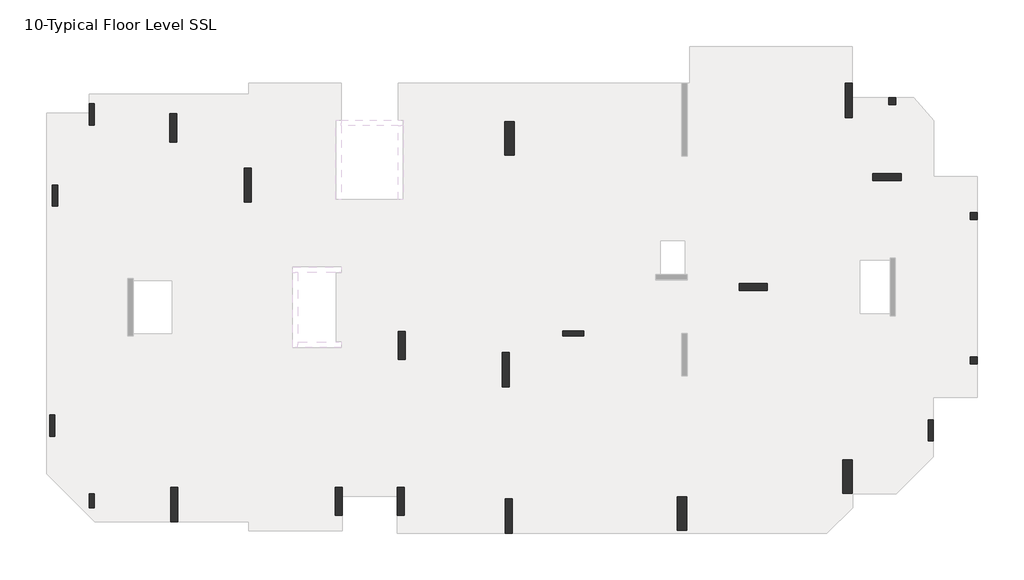
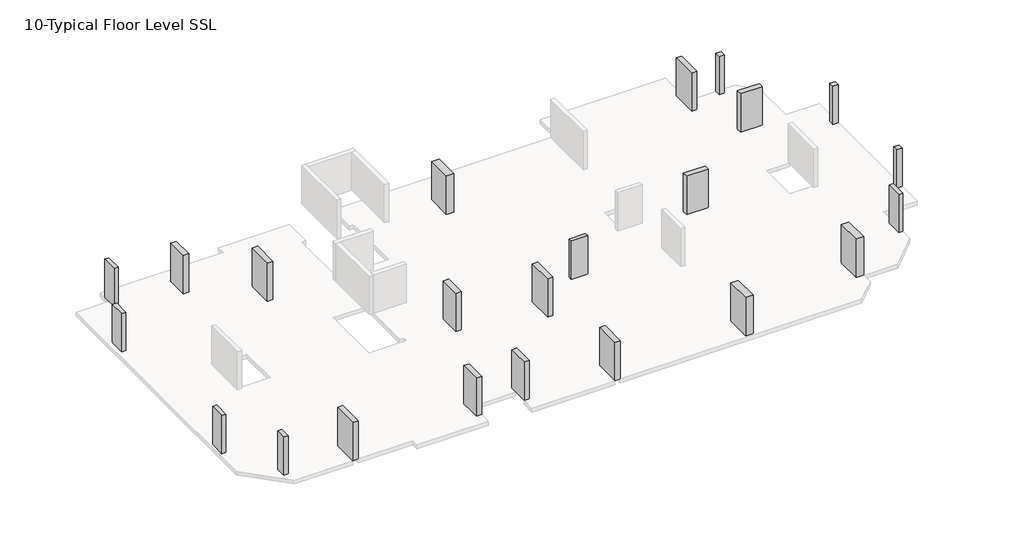
# One storey, part 2 of 2: 23 columns.
"""IFC4 building model written with IfcOpenShell, lengths in millimetres."""

import ifcopenshell
import ifcopenshell.guid

model = None  # the IFC model being written
_history = None  # IfcOwnerHistory: only IFC2X3 demands one
_inside = {}  # id of a spatial element -> (the spatial element, [elements in it])
_under = {}  # id of a project, library or spatial element -> (it, [spatial elements below it])
_declared = {}  # id of a project -> (the project, [libraries it declares])
_typed = {}  # id of a type object -> (the type object, [elements of that type])
_made_of = {}  # id of a material, layer set ... -> (it, [elements and type objects made of it])


def new_model(schema):
    """Start an empty IFC model of exactly this schema.

    Asked for "IFC4X3", IfcOpenShell would pick the latest addendum, in which some entities
    have other attributes; the version numbers below select the first issue.
    IFC2X3 requires an IfcOwnerHistory on every rooted entity: one is made here for all.
    """
    global model, _history
    if schema == "IFC4X3":
        model = ifcopenshell.file(schema_version=(4, 3, 0, 0))
    else:
        model = ifcopenshell.file(schema=schema)
    _inside.clear()
    _under.clear()
    _declared.clear()
    _typed.clear()
    _made_of.clear()
    _history = None
    if model.schema == "IFC2X3":
        org = make("IfcOrganization", Name="unknown")
        user = make(
            "IfcPersonAndOrganization",
            ThePerson=make("IfcPerson", FamilyName="unknown"),
            TheOrganization=org,
        )
        app = make(
            "IfcApplication",
            ApplicationDeveloper=org,
            Version="unknown",
            ApplicationFullName="unknown",
            ApplicationIdentifier="unknown",
        )
        _history = make(
            "IfcOwnerHistory",
            OwningUser=user,
            OwningApplication=app,
            ChangeAction="ADDED",
            CreationDate=0,
        )
    return model


def make(cls, **values):
    """One entity of the class cls with the attributes given. An attribute that is None is left unset."""
    return model.create_entity(
        cls, **{name: value for name, value in values.items() if value is not None}
    )


def rooted(cls, **values):
    """An entity with a GlobalId (a new one), such as an element, a storey or a relation."""
    return make(cls, GlobalId=ifcopenshell.guid.new(), OwnerHistory=_history, **values)


def si_unit(unit_type, name, prefix=None):
    """IfcSIUnit, for example si_unit("LENGTHUNIT", "METRE", prefix="MILLI")."""
    return make("IfcSIUnit", UnitType=unit_type, Prefix=prefix, Name=name)


def assignment(units):
    """IfcUnitAssignment: the units of a project."""
    return None if units is None else make("IfcUnitAssignment", Units=units)


def point(xyz):
    """IfcCartesianPoint."""
    return None if xyz is None else make("IfcCartesianPoint", Coordinates=xyz)


def direction(xyz):
    """IfcDirection."""
    return None if xyz is None else make("IfcDirection", DirectionRatios=xyz)


def frame(location, z_axis=None, x_axis=None):
    """IfcAxis2Placement3D, a coordinate frame: its origin and axes. An axis left out is left unset."""
    return make(
        "IfcAxis2Placement3D",
        Location=point(location),
        Axis=direction(z_axis),
        RefDirection=direction(x_axis),
    )


def origin():
    """The frame at (0, 0, 0) with its axes left unset."""
    return frame((0.0, 0.0, 0.0))


def place(relative_to, where):
    """IfcLocalPlacement: puts the frame where relative to a parent placement (None: the world)."""
    return make(
        "IfcLocalPlacement", PlacementRelTo=relative_to, RelativePlacement=where
    )


def context(
    kind, dimensions, precision=None, world=None, true_north=None, identifier=None
):
    """IfcGeometricRepresentationContext, for example the 3D "Model" context."""
    return make(
        "IfcGeometricRepresentationContext",
        ContextIdentifier=identifier,
        ContextType=kind,
        CoordinateSpaceDimension=dimensions,
        Precision=precision,
        WorldCoordinateSystem=world,
        TrueNorth=true_north,
    )


def project(units=None, contexts=None):
    """IfcProject with its units and contexts."""
    return rooted(
        "IfcProject",
        Name="project",
        RepresentationContexts=contexts,
        UnitsInContext=assignment(units),
    )


def spatial(cls, under=None, at=None, **own):
    """A site, building, storey or space (cls), placed at a placement, below another one or the project."""
    s = rooted(cls, ObjectPlacement=at, **own)
    if under is not None:
        _under.setdefault(under.id(), (under, []))[1].append(s)
    return s


def faces_of(points, faces, orient=None, outer=None):
    """IfcFace entities. A face is a list of loops; a loop is a list of indices into points, from 0.

    orient and outer hold one flag for each loop. By default every Orientation is true, the
    first loop of a face is its IfcFaceOuterBound and the others are IfcFaceBound.
    """
    made = []
    for i, loops in enumerate(faces):
        bounds = []
        for j, loop in enumerate(loops):
            is_outer = j == 0 if outer is None else outer[i][j]
            bounds.append(
                make(
                    "IfcFaceOuterBound" if is_outer else "IfcFaceBound",
                    Bound=make("IfcPolyLoop", Polygon=[points[k] for k in loop]),
                    Orientation=True if orient is None else orient[i][j],
                )
            )
        made.append(make("IfcFace", Bounds=bounds))
    return made


def faceted_brep(points, faces, orient=None, outer=None, voids=None):
    """IfcFacetedBrep: a solid bounded by flat faces; with voids (closed shells), ...WithVoids."""
    shared = [point(p) for p in points]
    hull = make("IfcClosedShell", CfsFaces=faces_of(shared, faces, orient, outer))
    if voids is None:
        return make("IfcFacetedBrep", Outer=hull)
    return make(
        "IfcFacetedBrepWithVoids",
        Outer=hull,
        Voids=[
            make(cls, CfsFaces=faces_of(shared, fs, o, b)) for cls, fs, o, b in voids
        ],
    )


def shape(context_of_items, identifier, shape_type, items):
    """IfcShapeRepresentation: the items that make up one representation, for example the "Body"."""
    return make(
        "IfcShapeRepresentation",
        ContextOfItems=context_of_items,
        RepresentationIdentifier=identifier,
        RepresentationType=shape_type,
        Items=items,
    )


def made_of(thing, what):
    """Note that an element or type object is made of a material, layer set ...; save() writes the relation."""
    if what is not None:
        _made_of.setdefault(what.id(), (what, []))[1].append(thing)
    return thing


def element(
    cls,
    number,
    at=None,
    inside=None,
    cuts=None,
    type_object=None,
    material=None,
    context=None,
    identifier="Body",
    shape_type=None,
    held_by="IfcProductDefinitionShape",
    body=None,
    shapes=None,
    **own,
):
    """One element of the class cls, such as IfcWall. Its Tag is "e" and its number.

    at: its placement. inside: the storey or other place that contains it. cuts: it is an
    opening in that element (IfcRelVoidsElement). A single representation is given by context,
    identifier, shape_type and body (its items); several are given by shapes. held_by: the class
    of the entity that holds the representations. save() writes the other relations.
    """
    e = rooted(cls, Tag="e%d" % number, ObjectPlacement=at, **own)
    if body is not None:
        shapes = [shape(context, identifier, shape_type, body)]
    if shapes is not None:
        e.Representation = make(held_by, Representations=shapes)
    if inside is not None:
        _inside.setdefault(inside.id(), (inside, []))[1].append(e)
    if cuts is not None:
        rooted(
            "IfcRelVoidsElement", RelatingBuildingElement=cuts, RelatedOpeningElement=e
        )
    if type_object is not None:
        _typed.setdefault(type_object.id(), (type_object, []))[1].append(e)
    return made_of(e, material)


def aggregate(whole, parts):
    """IfcRelAggregates: a whole, such as a stair, and the parts it consists of."""
    return rooted("IfcRelAggregates", RelatingObject=whole, RelatedObjects=parts)


def save(model, path):
    """Write the relations noted so far, then the file.

    IfcRelAggregates (storeys below a building ...), IfcRelContainedInSpatialStructure (elements
    in a storey), IfcRelDefinesByType, IfcRelAssociatesMaterial and IfcRelDeclares: one each for
    every whole, place, type object, material and project.
    """
    for whole, parts in _under.values():
        aggregate(whole, parts)
    for where, things in _inside.values():
        rooted(
            "IfcRelContainedInSpatialStructure",
            RelatedElements=things,
            RelatingStructure=where,
        )
    for kind, things in _typed.values():
        rooted("IfcRelDefinesByType", RelatedObjects=things, RelatingType=kind)
    for what, things in _made_of.values():
        rooted("IfcRelAssociatesMaterial", RelatedObjects=things, RelatingMaterial=what)
    for by, libraries in _declared.values():
        rooted("IfcRelDeclares", RelatingContext=by, RelatedDefinitions=libraries)
    model.write(path)


model = new_model("IFC4")

# Units and contexts
model_context = context("Model", 3, world=origin())
ifc_project = project(units=[si_unit("LENGTHUNIT", "METRE", prefix="MILLI")], contexts=[model_context])

# Site, building, storey
site = spatial("IfcSite", under=ifc_project)
building = spatial("IfcBuilding", under=site)
storey = spatial("IfcBuildingStorey", under=building, Name="10-Typical Floor Level SSL", Elevation=24000.0)

# Columns
placement = place(None, origin())
element("IfcColumn", 1, ObjectType="M_Concrete-Rectangular-Column : C-1 (400 x 400mm)", at=placement, inside=storey, context=model_context, shape_type="Brep", body=[
    faceted_brep([(52549.9999998, 16712.0, 24000.0), (52549.9999998, 16312.0, 24000.0), (52149.9999998, 16312.0, 24000.0), (52149.9999998, 16712.0, 24000.0), (52549.9999998, 16712.0, 27000.0), (52549.9999998, 16312.0, 27000.0), (52549.9999998, 16312.0, 26700.0), (52549.9999998, 16712.0, 26700.0), (52149.9999998, 16312.0, 27000.0), (52149.9999998, 16312.0, 26700.0), (52149.9999998, 16712.0, 27000.0), (52149.9999998, 16712.0, 26700.0)], [[[0, 1, 2, 3]], [[4, 5, 6, 1, 0, 7]], [[5, 8, 9, 2, 1, 6]], [[8, 10, 11, 3, 2, 9]], [[10, 4, 7, 0, 3, 11]], [[4, 10, 8, 5]]]),
])
element("IfcColumn", 2, ObjectType="M_Concrete-Rectangular-Column : C-1 (400 x 400mm)", at=placement, inside=storey, context=model_context, shape_type="Brep", body=[
    faceted_brep([(47898.6337868, 23252.0, 24000.0), (47898.6337868, 22852.0, 24000.0), (47498.6337868, 22852.0, 24000.0), (47498.6337868, 23252.0, 24000.0), (47898.6337868, 23252.0, 27000.0), (47898.6337868, 22852.0, 27000.0), (47898.6337868, 22852.0, 26700.0), (47498.6337868, 22852.0, 27000.0), (47498.6337868, 22852.0, 26700.0), (47498.6337868, 23252.0, 27000.0)], [[[0, 1, 2, 3]], [[4, 5, 6, 1, 0]], [[5, 7, 8, 2, 1, 6]], [[7, 9, 3, 2, 8]], [[9, 4, 0, 3]], [[4, 9, 7, 5]]]),
])
element("IfcColumn", 3, ObjectType="M_Concrete-Rectangular-Column : C-1 (400 x 400mm)", at=placement, inside=storey, context=model_context, shape_type="Brep", body=[
    faceted_brep([(52549.9999998, 8504.0039609, 24000.0), (52549.9999998, 8104.0039609, 24000.0), (52149.9999998, 8104.0039609, 24000.0), (52149.9999998, 8504.0039609, 24000.0), (52549.9999998, 8504.0039609, 27000.0), (52549.9999998, 8104.0039609, 27000.0), (52549.9999998, 8104.0039609, 26700.0), (52549.9999998, 8504.0039609, 26700.0), (52149.9999998, 8104.0039609, 27000.0), (52149.9999998, 8104.0039609, 26700.0), (52149.9999998, 8504.0039609, 27000.0), (52149.9999998, 8504.0039609, 26700.0)], [[[0, 1, 2, 3]], [[4, 5, 6, 1, 0, 7]], [[5, 8, 9, 2, 1, 6]], [[8, 10, 11, 3, 2, 9]], [[10, 4, 7, 0, 3, 11]], [[4, 10, 8, 5]]]),
])
element("IfcColumn", 4, ObjectType="M_Concrete-Rectangular-Column : C-2 (300 x 800mm)", at=placement, inside=storey, context=model_context, shape_type="Brep", body=[
    faceted_brep([(2352.0, 728.0, 24000.0), (2352.0, -72.0, 24000.0), (2052.0, -72.0, 24000.0), (2052.0, 728.0, 24000.0), (2352.0, 728.0, 27000.0), (2352.0, -72.0, 27000.0), (2352.0, -72.0, 26700.0), (2352.0, 728.0, 26700.0), (2052.0, -72.0, 27000.0), (2052.0, -72.0, 26700.0), (2052.0, 728.0, 27000.0), (2052.0, 728.0, 26700.0)], [[[0, 1, 2, 3]], [[4, 5, 6, 1, 0, 7]], [[5, 8, 9, 2, 1, 6]], [[8, 10, 11, 3, 2, 9]], [[10, 4, 7, 0, 3, 11]], [[4, 10, 8, 5]]]),
])
element("IfcColumn", 5, ObjectType="M_Concrete-Rectangular-Column : C-3(300 x 1200mm)", at=placement, inside=storey, context=model_context, shape_type="Brep", body=[
    faceted_brep([(2352.0, 22908.0000656, 24000.0), (2352.0, 21708.0000656, 24000.0), (2052.0, 21708.0000656, 24000.0), (2052.0, 22908.0000656, 24000.0), (2352.0, 22908.0000656, 27000.0), (2352.0, 21708.0000656, 27000.0), (2352.0, 21708.0000656, 26700.0), (2352.0, 22908.0000656, 26700.0), (2052.0, 21708.0000656, 27000.0), (2052.0, 21708.0000656, 26700.0), (2052.0, 22380.0004589, 27000.0), (2052.0, 22908.0000656, 27000.0), (2052.0, 22908.0000656, 26700.0)], [[[0, 1, 2, 3]], [[4, 5, 6, 1, 0, 7]], [[5, 8, 9, 2, 1, 6]], [[8, 10, 11, 12, 3, 2, 9]], [[11, 4, 7, 0, 3, 12]], [[4, 11, 10, 8, 5]]]),
])
element("IfcColumn", 6, ObjectType="M_Concrete-Rectangular-Column : C-3(300 x 1200mm)", at=placement, inside=storey, context=model_context, shape_type="Brep", body=[
    faceted_brep([(257.9999999, 18288.0, 24000.0), (257.9999999, 17088.0, 24000.0), (-42.0000001, 17088.0, 24000.0), (-42.0000001, 18288.0, 24000.0), (257.9999999, 18288.0, 27000.0), (257.9999999, 17088.0, 27000.0), (257.9999999, 17088.0, 26700.0), (257.9999999, 18288.0, 26700.0), (-42.0000001, 17088.0, 27000.0), (-42.0000001, 17088.0, 26700.0), (-42.0000001, 18288.0, 27000.0), (-42.0000001, 18288.0, 26700.0)], [[[0, 1, 2, 3]], [[4, 5, 6, 1, 0, 7]], [[5, 8, 9, 2, 1, 6]], [[8, 10, 11, 3, 2, 9]], [[10, 4, 7, 0, 3, 11]], [[4, 10, 8, 5]]]),
])
element("IfcColumn", 7, ObjectType="M_Concrete-Rectangular-Column : C-3(300 x 1200mm)", at=placement, inside=storey, context=model_context, shape_type="Brep", body=[
    faceted_brep([(108.001803, 5201.9999858, 24000.0), (108.001803, 4001.9999858, 24000.0), (-191.998197, 4001.9999858, 24000.0), (-191.998197, 5201.9999858, 24000.0), (108.001803, 5201.9999858, 27000.0), (108.001803, 4001.9999858, 27000.0), (108.001803, 4001.9999858, 26700.0), (108.001803, 5201.9999858, 26700.0), (-191.998197, 4001.9999858, 27000.0), (-191.998197, 4001.9999858, 26700.0), (-191.998197, 5201.9999858, 27000.0), (-191.998197, 5201.9999858, 26700.0)], [[[0, 1, 2, 3]], [[4, 5, 6, 1, 0, 7]], [[5, 8, 9, 2, 1, 6]], [[8, 10, 11, 3, 2, 9]], [[10, 4, 7, 0, 3, 11]], [[4, 10, 8, 5]]]),
])
element("IfcColumn", 8, ObjectType="M_Concrete-Rectangular-Column : C-3(300 x 1200mm)", at=placement, inside=storey, context=model_context, shape_type="Brep", body=[
    faceted_brep([(50046.0009271, 4931.9999929, 24000.0), (50046.0009271, 3731.9999929, 24000.0), (49746.0009271, 3731.9999929, 24000.0), (49746.0009271, 4931.9999929, 24000.0), (50046.0009271, 4931.9999929, 27000.0), (50046.0009271, 3731.9999929, 27000.0), (50046.0009271, 3731.9999929, 26700.0), (50046.0009271, 4931.9999929, 26700.0), (49746.0009271, 3731.9999929, 27000.0), (49746.0009271, 3731.9999929, 26700.0), (49746.0009271, 4931.9999929, 27000.0), (49746.0009271, 4931.9999929, 26700.0)], [[[0, 1, 2, 3]], [[4, 5, 6, 1, 0, 7]], [[5, 8, 9, 2, 1, 6]], [[8, 10, 11, 3, 2, 9]], [[10, 4, 7, 0, 3, 11]], [[4, 10, 8, 5]]]),
])
element("IfcColumn", 9, ObjectType="M_Concrete-Rectangular-Column : C-3(300 x 1200mm)", at=placement, inside=storey, context=model_context, shape_type="Brep", body=[
    faceted_brep([(28975.9999998, 9996.0000019, 24000.0), (30175.9999998, 9996.0000019, 24000.0), (30175.9999998, 9696.0000019, 24000.0), (28975.9999998, 9696.0000019, 24000.0), (28975.9999998, 9996.0000019, 27000.0), (30175.9999998, 9996.0000019, 27000.0), (30175.9999998, 9996.0000019, 26700.0), (28975.9999998, 9996.0000019, 26700.0), (30175.9999998, 9696.0000019, 27000.0), (30175.9999998, 9696.0000019, 26700.0), (28975.9999998, 9696.0000019, 27000.0), (28975.9999998, 9696.0000019, 26700.0)], [[[0, 1, 2, 3]], [[4, 5, 6, 1, 0, 7]], [[5, 8, 9, 2, 1, 6]], [[8, 10, 11, 3, 2, 9]], [[10, 4, 7, 0, 3, 11]], [[4, 10, 8, 5]]]),
])
element("IfcColumn", 10, ObjectType="M_Concrete-Rectangular-Column : C-4 (400 x 1600mm)", at=placement, inside=storey, context=model_context, shape_type="Brep", body=[
    faceted_brep([(7021.9999999, 22340.0000078, 24000.0), (7021.9999999, 20740.0000078, 24000.0), (6621.9999999, 20740.0000078, 24000.0), (6621.9999999, 22340.0000078, 24000.0), (7021.9999999, 22340.0000078, 27000.0), (7021.9999999, 20740.0000078, 27000.0), (7021.9999999, 20740.0000078, 26700.0), (7021.9999999, 22340.0000078, 26700.0), (6621.9999999, 20740.0000078, 27000.0), (6621.9999999, 20740.0000078, 26700.0), (6621.9999999, 22340.0000078, 27000.0), (6621.9999999, 22340.0000078, 26700.0)], [[[0, 1, 2, 3]], [[4, 5, 6, 1, 0, 7]], [[5, 8, 9, 2, 1, 6]], [[8, 10, 11, 3, 2, 9]], [[10, 4, 7, 0, 3, 11]], [[4, 10, 8, 5]]]),
])
element("IfcColumn", 11, ObjectType="M_Concrete-Rectangular-Column : C-4 (400 x 1600mm)", at=placement, inside=storey, context=model_context, shape_type="Brep", body=[
    faceted_brep([(19969.9997488, 1087.9955348, 24000.0), (19969.9997488, -512.0044652, 24000.0), (19569.9997488, -512.0044652, 24000.0), (19569.9997488, 1087.9955348, 24000.0), (19969.9997488, 1087.9955348, 27000.0), (19969.9997488, -512.0044652, 27000.0), (19969.9997488, -512.0044652, 26700.0), (19969.9997488, 1087.9955348, 26700.0), (19569.9997488, -512.0044652, 27000.0), (19569.9997488, -512.0044652, 26700.0), (19569.9997488, 564.000519, 27000.0), (19569.9997488, 1087.9955348, 27000.0), (19569.9997488, 1087.9955348, 26700.0)], [[[0, 1, 2, 3]], [[4, 5, 6, 1, 0, 7]], [[5, 8, 9, 2, 1, 6]], [[8, 10, 11, 12, 3, 2, 9]], [[11, 4, 7, 0, 3, 12]], [[4, 11, 10, 8, 5]]]),
])
element("IfcColumn", 12, ObjectType="M_Concrete-Rectangular-Column : C-4 (400 x 1600mm)", at=placement, inside=storey, context=model_context, shape_type="Brep", body=[
    faceted_brep([(46605.9993605, 18950.0, 24000.0), (48205.9993605, 18950.0, 24000.0), (48205.9993605, 18550.0, 24000.0), (46605.9993605, 18550.0, 24000.0), (46605.9993605, 18950.0, 27000.0), (48205.9993605, 18950.0, 27000.0), (48205.9993605, 18950.0, 26700.0), (46605.9993605, 18950.0, 26700.0), (48205.9993605, 18550.0, 27000.0), (48205.9993605, 18550.0, 26700.0), (46605.9993605, 18550.0, 27000.0), (46605.9993605, 18550.0, 26700.0)], [[[0, 1, 2, 3]], [[4, 5, 6, 1, 0, 7]], [[5, 8, 9, 2, 1, 6]], [[8, 10, 11, 3, 2, 9]], [[10, 4, 7, 0, 3, 11]], [[4, 10, 8, 5]]]),
])
element("IfcColumn", 13, ObjectType="M_Concrete-Rectangular-Column : C-5 (400 x 1600mm)", at=placement, inside=storey, context=model_context, shape_type="Brep", body=[
    faceted_brep([(20030.000009, 9955.9999979, 24000.0), (20030.000009, 8355.9999979, 24000.0), (19630.000009, 8355.9999979, 24000.0), (19630.000009, 9955.9999979, 24000.0), (20030.000009, 9955.9999979, 27000.0), (20030.000009, 8355.9999979, 27000.0), (20030.000009, 8355.9999979, 26700.0), (20030.000009, 9955.9999979, 26700.0), (19630.000009, 8355.9999979, 27000.0), (19630.000009, 8355.9999979, 26700.0), (19630.000009, 9955.9999979, 27000.0), (19630.000009, 9955.9999979, 26700.0)], [[[0, 1, 2, 3]], [[4, 5, 6, 1, 0, 7]], [[5, 8, 9, 2, 1, 6]], [[8, 10, 11, 3, 2, 9]], [[10, 4, 7, 0, 3, 11]], [[4, 10, 8, 5]]]),
])
element("IfcColumn", 14, ObjectType="M_Concrete-Rectangular-Column : C-5 (400 x 1600mm)", at=placement, inside=storey, context=model_context, shape_type="Brep", body=[
    faceted_brep([(16429.9999981, 1088.0, 24000.0), (16429.9999981, -512.0, 24000.0), (16029.9999981, -512.0, 24000.0), (16029.9999981, 1088.0, 24000.0), (16429.9999981, 1088.0, 27000.0), (16429.9999981, 564.000519, 27000.0), (16429.9999981, -512.0, 27000.0), (16429.9999981, -512.0, 26700.0), (16429.9999981, 1088.0, 26700.0), (16029.9999981, -512.0, 27000.0), (16029.9999981, -512.0, 26700.0), (16029.9999981, 1088.0, 27000.0), (16029.9999981, 1088.0, 26700.0)], [[[0, 1, 2, 3]], [[4, 5, 6, 7, 1, 0, 8]], [[6, 9, 10, 2, 1, 7]], [[9, 11, 12, 3, 2, 10]], [[11, 4, 8, 0, 3, 12]], [[4, 11, 9, 6, 5]]]),
])
element("IfcColumn", 15, ObjectType="M_Concrete-Rectangular-Column : C-5 (400 x 1600mm)", at=placement, inside=storey, context=model_context, shape_type="Brep", body=[
    faceted_brep([(38998.0014887, 12692.0079212, 24000.0), (40598.0014887, 12692.0079212, 24000.0), (40598.0014887, 12292.0079212, 24000.0), (38998.0014887, 12292.0079212, 24000.0), (38998.0014887, 12692.0079212, 27000.0), (40598.0014887, 12692.0079212, 27000.0), (40598.0014887, 12692.0079212, 26700.0), (38998.0014887, 12692.0079212, 26700.0), (40598.0014887, 12292.0079212, 27000.0), (40598.0014887, 12292.0079212, 26700.0), (38998.0014887, 12292.0079212, 27000.0), (38998.0014887, 12292.0079212, 26700.0)], [[[0, 1, 2, 3]], [[4, 5, 6, 1, 0, 7]], [[5, 8, 9, 2, 1, 6]], [[8, 10, 11, 3, 2, 9]], [[10, 4, 7, 0, 3, 11]], [[4, 10, 8, 5]]]),
])
element("IfcColumn", 16, ObjectType="M_Concrete-Rectangular-Column : C-6 (400 x 1950mm)", at=placement, inside=storey, context=model_context, shape_type="Brep", body=[
    faceted_brep([(11270.0000427, 19262.9999996, 24000.0), (11270.0000427, 17312.9999996, 24000.0), (10870.0000427, 17312.9999996, 24000.0), (10870.0000427, 19262.9999996, 24000.0), (11270.0000427, 19262.9999996, 27000.0), (11270.0000427, 17312.9999996, 27000.0), (11270.0000427, 17312.9999996, 26700.0), (11270.0000427, 19262.9999996, 26700.0), (10870.0000427, 17312.9999996, 27000.0), (10870.0000427, 17312.9999996, 26700.0), (10870.0000427, 19262.9999996, 27000.0), (10870.0000427, 19262.9999996, 26700.0)], [[[0, 1, 2, 3]], [[4, 5, 6, 1, 0, 7]], [[5, 8, 9, 2, 1, 6]], [[8, 10, 11, 3, 2, 9]], [[10, 4, 7, 0, 3, 11]], [[4, 10, 8, 5]]]),
])
element("IfcColumn", 17, ObjectType="M_Concrete-Rectangular-Column : C-6 (400 x 1950mm)", at=placement, inside=storey, context=model_context, shape_type="Brep", body=[
    faceted_brep([(7082.0000416, 1083.0000153, 24000.0), (7082.0000416, -866.9999847, 24000.0), (6682.0000416, -866.9999847, 24000.0), (6682.0000416, 1083.0000153, 24000.0), (7082.0000416, 1083.0000153, 27000.0), (7082.0000416, -866.9999847, 27000.0), (7082.0000416, -866.9999847, 26700.0), (7082.0000416, 1083.0000153, 26700.0), (6682.0000416, -866.9999847, 27000.0), (6682.0000416, -866.9999847, 26700.0), (6682.0000416, 1083.0000153, 27000.0), (6682.0000416, 1083.0000153, 26700.0)], [[[0, 1, 2, 3]], [[4, 5, 6, 1, 0, 7]], [[5, 8, 9, 2, 1, 6]], [[8, 10, 11, 3, 2, 9]], [[10, 4, 7, 0, 3, 11]], [[4, 10, 8, 5]]]),
])
element("IfcColumn", 18, ObjectType="M_Concrete-Rectangular-Column : C-6 (400 x 1950mm)", at=placement, inside=storey, context=model_context, shape_type="Brep", body=[
    faceted_brep([(26113.9999998, 422.995535, 24000.0), (26113.9999998, -1527.004465, 24000.0), (25713.9999998, -1527.004465, 24000.0), (25713.9999998, 422.995535, 24000.0), (26113.9999998, 422.995535, 27000.0), (26113.9999998, -1527.004465, 27000.0), (26113.9999998, -1527.004465, 26700.0), (26113.9999998, 422.995535, 26700.0), (25713.9999998, -1527.004465, 27000.0), (25713.9999998, -1527.004465, 26700.0), (25713.9999998, 422.995535, 27000.0), (25713.9999998, 422.995535, 26700.0)], [[[0, 1, 2, 3]], [[4, 5, 6, 1, 0, 7]], [[5, 8, 9, 2, 1, 6]], [[8, 10, 11, 3, 2, 9]], [[10, 4, 7, 0, 3, 11]], [[4, 10, 8, 5]]]),
])
element("IfcColumn", 19, ObjectType="M_Concrete-Rectangular-Column : C-6 (400 x 1950mm)", at=placement, inside=storey, context=model_context, shape_type="Brep", body=[
    faceted_brep([(45446.0007483, 24087.0, 24000.0), (45446.0007483, 22137.0, 24000.0), (45046.0007483, 22137.0, 24000.0), (45046.0007483, 24087.0, 24000.0), (45446.0007483, 24087.0, 27000.0), (45446.0007483, 23252.0000315, 27000.0), (45446.0007483, 22137.0, 27000.0), (45446.0007483, 22137.0, 26700.0), (45446.0007483, 24087.0, 26700.0), (45046.0007483, 22137.0, 27000.0), (45046.0007483, 22137.0, 26700.0), (45046.0007483, 24087.0, 27000.0), (45046.0007483, 24087.0, 26700.0)], [[[0, 1, 2, 3]], [[4, 5, 6, 7, 1, 0, 8]], [[6, 9, 10, 2, 1, 7]], [[9, 11, 12, 3, 2, 10]], [[11, 4, 8, 0, 3, 12]], [[4, 11, 9, 6, 5]]]),
])
element("IfcColumn", 20, ObjectType="M_Concrete-Rectangular-Column : C-6 (400 x 1950mm)", at=placement, inside=storey, context=model_context, shape_type="Brep", body=[
    faceted_brep([(25934.0000455, 8751.0001824, 24000.0), (25934.0000455, 6801.0001824, 24000.0), (25534.0000455, 6801.0001824, 24000.0), (25534.0000455, 8751.0001824, 24000.0), (25934.0000455, 8751.0001824, 27000.0), (25934.0000455, 6801.0001824, 27000.0), (25934.0000455, 6801.0001824, 26700.0), (25934.0000455, 8751.0001824, 26700.0), (25534.0000455, 6801.0001824, 27000.0), (25534.0000455, 6801.0001824, 26700.0), (25534.0000455, 8751.0001824, 27000.0), (25534.0000455, 8751.0001824, 26700.0)], [[[0, 1, 2, 3]], [[4, 5, 6, 1, 0, 7]], [[5, 8, 9, 2, 1, 6]], [[8, 10, 11, 3, 2, 9]], [[10, 4, 7, 0, 3, 11]], [[4, 10, 8, 5]]]),
])
element("IfcColumn", 21, ObjectType="M_Concrete-Rectangular-Column : C-7 (550 x 1900mm)", at=placement, inside=storey, context=model_context, shape_type="Brep", body=[
    faceted_brep([(36035.9999998, 548.0007983, 24000.0), (36035.9999998, -1351.9992017, 24000.0), (35485.9999998, -1351.9992017, 24000.0), (35485.9999998, 548.0007983, 24000.0), (36035.9999998, 548.0007983, 27000.0), (36035.9999998, -1351.9992017, 27000.0), (36035.9999998, -1351.9992017, 26700.0), (36035.9999998, 548.0007983, 26700.0), (35485.9999998, -1351.9992017, 27000.0), (35485.9999998, -1351.9992017, 26700.0), (35485.9999998, 548.0007983, 27000.0), (35485.9999998, 548.0007983, 26700.0)], [[[0, 1, 2, 3]], [[4, 5, 6, 1, 0, 7]], [[5, 8, 9, 2, 1, 6]], [[8, 10, 11, 3, 2, 9]], [[10, 4, 7, 0, 3, 11]], [[4, 10, 8, 5]]]),
])
element("IfcColumn", 22, ObjectType="M_Concrete-Rectangular-Column : C-7 (550 x 1900mm)", at=placement, inside=storey, context=model_context, shape_type="Brep", body=[
    faceted_brep([(45443.9999998, 2648.0, 24000.0), (45443.9999998, 748.0, 24000.0), (44893.9999998, 748.0, 24000.0), (44893.9999998, 2648.0, 24000.0), (45443.9999998, 2648.0, 27000.0), (45443.9999998, 748.0, 27000.0), (45443.9999998, 748.0, 26700.0), (45443.9999998, 2648.0, 26700.0), (44893.9999998, 748.0, 27000.0), (44893.9999998, 748.0, 26700.0), (44893.9999998, 2648.0, 27000.0), (44893.9999998, 2648.0, 26700.0)], [[[0, 1, 2, 3]], [[4, 5, 6, 1, 0, 7]], [[5, 8, 9, 2, 1, 6]], [[8, 10, 11, 3, 2, 9]], [[10, 4, 7, 0, 3, 11]], [[4, 10, 8, 5]]]),
])
element("IfcColumn", 23, ObjectType="M_Concrete-Rectangular-Column : C-7 (550 x 1900mm)", at=placement, inside=storey, context=model_context, shape_type="Brep", body=[
    faceted_brep([(26218.9999998, 21900.0, 24000.0), (26218.9999998, 20000.0, 24000.0), (25668.9999998, 20000.0, 24000.0), (25668.9999998, 21900.0, 24000.0), (26218.9999998, 21900.0, 27000.0), (26218.9999998, 20000.0, 27000.0), (26218.9999998, 20000.0, 26700.0), (26218.9999998, 21900.0, 26700.0), (25668.9999998, 20000.0, 27000.0), (25668.9999998, 20000.0, 26700.0), (25668.9999998, 21900.0, 27000.0), (25668.9999998, 21900.0, 26700.0)], [[[0, 1, 2, 3]], [[4, 5, 6, 1, 0, 7]], [[5, 8, 9, 2, 1, 6]], [[8, 10, 11, 3, 2, 9]], [[10, 4, 7, 0, 3, 11]], [[4, 10, 8, 5]]]),
])

save(model, "model.ifc")

# Revit data of these elements
# Type "M_Concrete-Rectangular-Column : C-1 (400 x 400mm)"
#   Type Mark = "C01"
#   b = 400 mm
#   h = 400 mm
#   Structural Material [instance default] = Concrete, Cast-in-Place gray
# Type "M_Concrete-Rectangular-Column : C-2 (300 x 800mm)"
#   Type Mark = "C02"
#   b = 300 mm
#   h = 800 mm
#   Structural Material [instance default] = Concrete, Cast-in-Place gray
# Type "M_Concrete-Rectangular-Column : C-3(300 x 1200mm)"
#   Type Mark = "C03"
#   b = 300 mm
#   h = 1200 mm
#   Structural Material [instance default] = Concrete, Cast-in-Place gray
# Type "M_Concrete-Rectangular-Column : C-4 (400 x 1600mm)"
#   Type Mark = "C04"
#   b = 400 mm
#   h = 1600 mm
#   Structural Material [instance default] = Concrete, Cast-in-Place gray
# Type "M_Concrete-Rectangular-Column : C-5 (400 x 1600mm)"
#   Type Mark = "C05"
#   b = 400 mm
#   h = 1600 mm
#   Structural Material [instance default] = Concrete, Cast-in-Place gray
# Type "M_Concrete-Rectangular-Column : C-6 (400 x 1950mm)"
#   Type Mark = "C06"
#   b = 400 mm
#   h = 1950 mm
#   Structural Material [instance default] = Concrete, Cast-in-Place gray
# Type "M_Concrete-Rectangular-Column : C-7 (550 x 1900mm)"
#   Type Mark = "C07"
#   b = 550 mm
#   h = 1900 mm
#   Structural Material [instance default] = Concrete, Cast-in-Place gray
# Elements 1, 2, 3 (IfcColumn, "M_Concrete-Rectangular-Column : C-1 (400 x 400mm)")
#   Structural Material = Concrete-RC
#   Phase Created = New Construction
#   Materials on its faces: "Concrete-RC"
# Element 4 (IfcColumn, "M_Concrete-Rectangular-Column : C-2 (300 x 800mm)")
#   Structural Material = Concrete-RC
#   Phase Created = New Construction
#   Materials on its faces: "Concrete-RC"
# Elements 5, 6, 7, 8, 9 (IfcColumn, "M_Concrete-Rectangular-Column : C-3(300 x 1200mm)")
#   Structural Material = Concrete-RC
#   Phase Created = New Construction
#   Materials on its faces: "Concrete-RC"
# Elements 10, 11, 12 (IfcColumn, "M_Concrete-Rectangular-Column : C-4 (400 x 1600mm)")
#   Structural Material = Concrete-RC
#   Phase Created = New Construction
#   Materials on its faces: "Concrete-RC"
# Elements 13, 14, 15 (IfcColumn, "M_Concrete-Rectangular-Column : C-5 (400 x 1600mm)")
#   Structural Material = Concrete-RC
#   Phase Created = New Construction
#   Materials on its faces: "Concrete-RC"
# Elements 16, 17, 18, 19, 20 (IfcColumn, "M_Concrete-Rectangular-Column : C-6 (400 x 1950mm)")
#   Structural Material = Concrete-RC
#   Phase Created = New Construction
#   Materials on its faces: "Concrete-RC"
# Elements 21, 22, 23 (IfcColumn, "M_Concrete-Rectangular-Column : C-7 (550 x 1900mm)")
#   Structural Material = Concrete-RC
#   Phase Created = New Construction
#   Materials on its faces: "Concrete-RC"
# Materials
#   "Concrete, Cast-in-Place gray": class "Concrete", colour RGB 192 192 192, transparency 0, Description = "Cast-in-place concrete", Cost = 0
#   "Concrete-RC": class "Concrete", colour RGB 128 128 128, transparency 0, Description = "High strength concrete", Cost = 0
